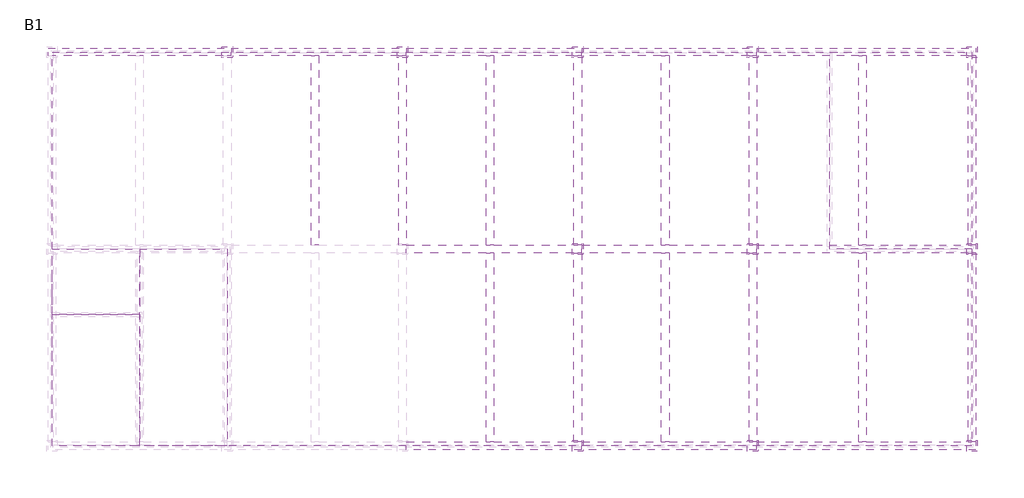
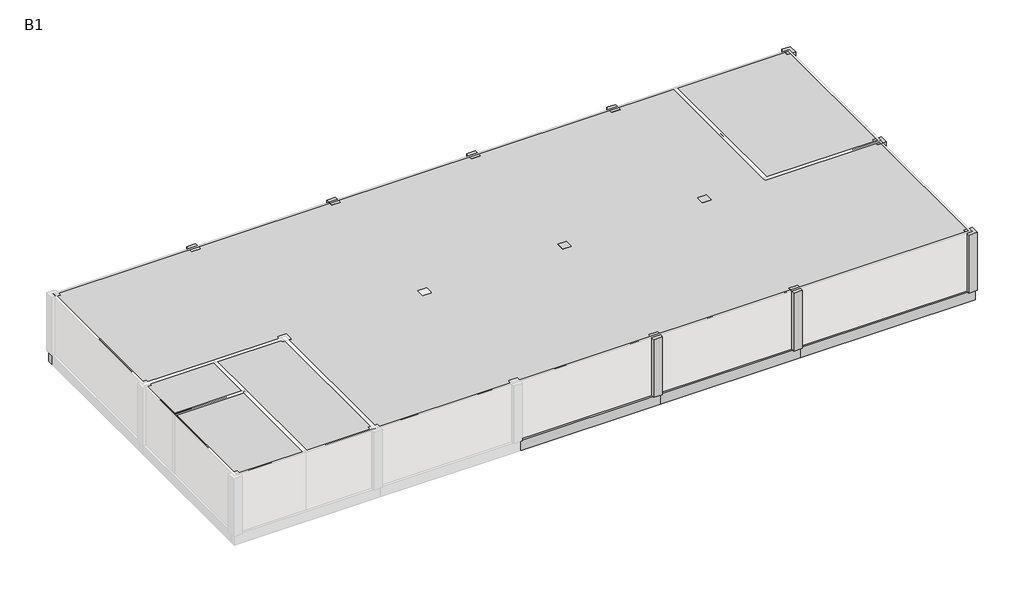
# One storey, part 2 of 2: 25 beams, 11 columns, 5 proxies.
"""IFC4 building model written with IfcOpenShell, lengths in millimetres."""

import ifcopenshell
import ifcopenshell.guid

model = None  # the IFC model being written
_history = None  # IfcOwnerHistory: only IFC2X3 demands one
_inside = {}  # id of a spatial element -> (the spatial element, [elements in it])
_under = {}  # id of a project, library or spatial element -> (it, [spatial elements below it])
_declared = {}  # id of a project -> (the project, [libraries it declares])
_typed = {}  # id of a type object -> (the type object, [elements of that type])
_made_of = {}  # id of a material, layer set ... -> (it, [elements and type objects made of it])


def new_model(schema):
    """Start an empty IFC model of exactly this schema.

    Asked for "IFC4X3", IfcOpenShell would pick the latest addendum, in which some entities
    have other attributes; the version numbers below select the first issue.
    IFC2X3 requires an IfcOwnerHistory on every rooted entity: one is made here for all.
    """
    global model, _history
    if schema == "IFC4X3":
        model = ifcopenshell.file(schema_version=(4, 3, 0, 0))
    else:
        model = ifcopenshell.file(schema=schema)
    _inside.clear()
    _under.clear()
    _declared.clear()
    _typed.clear()
    _made_of.clear()
    _history = None
    if model.schema == "IFC2X3":
        org = make("IfcOrganization", Name="unknown")
        user = make(
            "IfcPersonAndOrganization",
            ThePerson=make("IfcPerson", FamilyName="unknown"),
            TheOrganization=org,
        )
        app = make(
            "IfcApplication",
            ApplicationDeveloper=org,
            Version="unknown",
            ApplicationFullName="unknown",
            ApplicationIdentifier="unknown",
        )
        _history = make(
            "IfcOwnerHistory",
            OwningUser=user,
            OwningApplication=app,
            ChangeAction="ADDED",
            CreationDate=0,
        )
    return model


def make(cls, **values):
    """One entity of the class cls with the attributes given. An attribute that is None is left unset."""
    return model.create_entity(
        cls, **{name: value for name, value in values.items() if value is not None}
    )


def rooted(cls, **values):
    """An entity with a GlobalId (a new one), such as an element, a storey or a relation."""
    return make(cls, GlobalId=ifcopenshell.guid.new(), OwnerHistory=_history, **values)


def si_unit(unit_type, name, prefix=None):
    """IfcSIUnit, for example si_unit("LENGTHUNIT", "METRE", prefix="MILLI")."""
    return make("IfcSIUnit", UnitType=unit_type, Prefix=prefix, Name=name)


def assignment(units):
    """IfcUnitAssignment: the units of a project."""
    return None if units is None else make("IfcUnitAssignment", Units=units)


def point(xyz):
    """IfcCartesianPoint."""
    return None if xyz is None else make("IfcCartesianPoint", Coordinates=xyz)


def direction(xyz):
    """IfcDirection."""
    return None if xyz is None else make("IfcDirection", DirectionRatios=xyz)


def frame(location, z_axis=None, x_axis=None):
    """IfcAxis2Placement3D, a coordinate frame: its origin and axes. An axis left out is left unset."""
    return make(
        "IfcAxis2Placement3D",
        Location=point(location),
        Axis=direction(z_axis),
        RefDirection=direction(x_axis),
    )


def origin():
    """The frame at (0, 0, 0) with its axes left unset."""
    return frame((0.0, 0.0, 0.0))


def origin_with_axes():
    """The frame at (0, 0, 0) with the z axis (0, 0, 1) and the x axis (1, 0, 0) written out."""
    return frame((0.0, 0.0, 0.0), z_axis=(0.0, 0.0, 1.0), x_axis=(1.0, 0.0, 0.0))


def place(relative_to, where):
    """IfcLocalPlacement: puts the frame where relative to a parent placement (None: the world)."""
    return make(
        "IfcLocalPlacement", PlacementRelTo=relative_to, RelativePlacement=where
    )


def context(
    kind, dimensions, precision=None, world=None, true_north=None, identifier=None
):
    """IfcGeometricRepresentationContext, for example the 3D "Model" context."""
    return make(
        "IfcGeometricRepresentationContext",
        ContextIdentifier=identifier,
        ContextType=kind,
        CoordinateSpaceDimension=dimensions,
        Precision=precision,
        WorldCoordinateSystem=world,
        TrueNorth=true_north,
    )


def project(units=None, contexts=None):
    """IfcProject with its units and contexts."""
    return rooted(
        "IfcProject",
        Name="project",
        RepresentationContexts=contexts,
        UnitsInContext=assignment(units),
    )


def spatial(cls, under=None, at=None, **own):
    """A site, building, storey or space (cls), placed at a placement, below another one or the project."""
    s = rooted(cls, ObjectPlacement=at, **own)
    if under is not None:
        _under.setdefault(under.id(), (under, []))[1].append(s)
    return s


def polyline(points):
    """IfcPolyline through the points."""
    return make("IfcPolyline", Points=[point(p) for p in points])


def outline(outer, holes=None, kind="AREA"):
    """IfcArbitraryClosedProfileDef: a profile drawn as a closed curve; with holes, ...WithVoids."""
    if holes is None:
        return make("IfcArbitraryClosedProfileDef", ProfileType=kind, OuterCurve=outer)
    return make(
        "IfcArbitraryProfileDefWithVoids",
        ProfileType=kind,
        OuterCurve=outer,
        InnerCurves=holes,
    )


def extrude(swept, where, along, depth):
    """IfcExtrudedAreaSolid: the profile swept, set in the frame where, extruded along a direction by depth."""
    return make(
        "IfcExtrudedAreaSolid",
        SweptArea=swept,
        Position=where,
        ExtrudedDirection=direction(along),
        Depth=depth,
    )


def faces_of(points, faces, orient=None, outer=None):
    """IfcFace entities. A face is a list of loops; a loop is a list of indices into points, from 0.

    orient and outer hold one flag for each loop. By default every Orientation is true, the
    first loop of a face is its IfcFaceOuterBound and the others are IfcFaceBound.
    """
    made = []
    for i, loops in enumerate(faces):
        bounds = []
        for j, loop in enumerate(loops):
            is_outer = j == 0 if outer is None else outer[i][j]
            bounds.append(
                make(
                    "IfcFaceOuterBound" if is_outer else "IfcFaceBound",
                    Bound=make("IfcPolyLoop", Polygon=[points[k] for k in loop]),
                    Orientation=True if orient is None else orient[i][j],
                )
            )
        made.append(make("IfcFace", Bounds=bounds))
    return made


def faceted_brep(points, faces, orient=None, outer=None, voids=None):
    """IfcFacetedBrep: a solid bounded by flat faces; with voids (closed shells), ...WithVoids."""
    shared = [point(p) for p in points]
    hull = make("IfcClosedShell", CfsFaces=faces_of(shared, faces, orient, outer))
    if voids is None:
        return make("IfcFacetedBrep", Outer=hull)
    return make(
        "IfcFacetedBrepWithVoids",
        Outer=hull,
        Voids=[
            make(cls, CfsFaces=faces_of(shared, fs, o, b)) for cls, fs, o, b in voids
        ],
    )


def shape(context_of_items, identifier, shape_type, items):
    """IfcShapeRepresentation: the items that make up one representation, for example the "Body"."""
    return make(
        "IfcShapeRepresentation",
        ContextOfItems=context_of_items,
        RepresentationIdentifier=identifier,
        RepresentationType=shape_type,
        Items=items,
    )


def source(mapping_origin, context_of_items, identifier, shape_type, items):
    """IfcRepresentationMap: a shape defined once, which mapped items show again and again."""
    return make(
        "IfcRepresentationMap",
        MappingOrigin=mapping_origin,
        MappedRepresentation=shape(context_of_items, identifier, shape_type, items),
    )


def transform(
    local_origin,
    x_axis=None,
    y_axis=None,
    z_axis=None,
    scale=None,
    scale2=None,
    scale3=None,
    uniform=True,
):
    """IfcCartesianTransformationOperator3D, or its non-uniform kind. x_axis, y_axis, z_axis: its Axis1, 2, 3."""
    if uniform:
        return make(
            "IfcCartesianTransformationOperator3D",
            Axis1=direction(x_axis),
            Axis2=direction(y_axis),
            LocalOrigin=point(local_origin),
            Scale=scale,
            Axis3=direction(z_axis),
        )
    return make(
        "IfcCartesianTransformationOperator3DnonUniform",
        Axis1=direction(x_axis),
        Axis2=direction(y_axis),
        LocalOrigin=point(local_origin),
        Scale=scale,
        Axis3=direction(z_axis),
        Scale2=scale2,
        Scale3=scale3,
    )


def mapped(mapping_source, mapping_target):
    """IfcMappedItem: shows the shape of a source again, moved by a transform."""
    return make(
        "IfcMappedItem", MappingSource=mapping_source, MappingTarget=mapping_target
    )


def made_of(thing, what):
    """Note that an element or type object is made of a material, layer set ...; save() writes the relation."""
    if what is not None:
        _made_of.setdefault(what.id(), (what, []))[1].append(thing)
    return thing


def element(
    cls,
    number,
    at=None,
    inside=None,
    cuts=None,
    type_object=None,
    material=None,
    context=None,
    identifier="Body",
    shape_type=None,
    held_by="IfcProductDefinitionShape",
    body=None,
    shapes=None,
    **own,
):
    """One element of the class cls, such as IfcWall. Its Tag is "e" and its number.

    at: its placement. inside: the storey or other place that contains it. cuts: it is an
    opening in that element (IfcRelVoidsElement). A single representation is given by context,
    identifier, shape_type and body (its items); several are given by shapes. held_by: the class
    of the entity that holds the representations. save() writes the other relations.
    """
    e = rooted(cls, Tag="e%d" % number, ObjectPlacement=at, **own)
    if body is not None:
        shapes = [shape(context, identifier, shape_type, body)]
    if shapes is not None:
        e.Representation = make(held_by, Representations=shapes)
    if inside is not None:
        _inside.setdefault(inside.id(), (inside, []))[1].append(e)
    if cuts is not None:
        rooted(
            "IfcRelVoidsElement", RelatingBuildingElement=cuts, RelatedOpeningElement=e
        )
    if type_object is not None:
        _typed.setdefault(type_object.id(), (type_object, []))[1].append(e)
    return made_of(e, material)


def aggregate(whole, parts):
    """IfcRelAggregates: a whole, such as a stair, and the parts it consists of."""
    return rooted("IfcRelAggregates", RelatingObject=whole, RelatedObjects=parts)


def save(model, path):
    """Write the relations noted so far, then the file.

    IfcRelAggregates (storeys below a building ...), IfcRelContainedInSpatialStructure (elements
    in a storey), IfcRelDefinesByType, IfcRelAssociatesMaterial and IfcRelDeclares: one each for
    every whole, place, type object, material and project.
    """
    for whole, parts in _under.values():
        aggregate(whole, parts)
    for where, things in _inside.values():
        rooted(
            "IfcRelContainedInSpatialStructure",
            RelatedElements=things,
            RelatingStructure=where,
        )
    for kind, things in _typed.values():
        rooted("IfcRelDefinesByType", RelatedObjects=things, RelatingType=kind)
    for what, things in _made_of.values():
        rooted("IfcRelAssociatesMaterial", RelatedObjects=things, RelatingMaterial=what)
    for by, libraries in _declared.values():
        rooted("IfcRelDeclares", RelatingContext=by, RelatedDefinitions=libraries)
    model.write(path)


def generic_models_bb515c93(model_context):
    return source(origin(), model_context, "Body", "SweptSolid", [
        extrude(outline(polyline([(9000.0, 21000.0), (9000.0, -21000.0), (-9000.0, -21000.0), (-9000.0, 21000.0), (9000.0, 21000.0)])), origin_with_axes(), (0.0, 0.0, 1.0), 3500.0),
    ])


def generic_models_5926095e(model_context):
    return source(origin(), model_context, "Body", "SweptSolid", [
        extrude(outline(polyline([(3250.0, 4500.0), (3250.0, -4500.0), (-3250.0, -4500.0), (-3250.0, 4500.0), (3250.0, 4500.0)])), origin_with_axes(), (0.0, 0.0, 1.0), 3500.0),
    ])


def generic_models_0b067365(model_context):
    return source(origin(), model_context, "Body", "SweptSolid", [
        extrude(outline(polyline([(2000.0, 4500.0), (2000.0, -4500.0), (-2000.0, -4500.0), (-2000.0, 4500.0), (2000.0, 4500.0)])), origin_with_axes(), (0.0, 0.0, 1.0), 3500.0),
    ])


def generic_models_4c644d41(model_context):
    return source(origin(), model_context, "Body", "SweptSolid", [
        extrude(outline(polyline([(2000.0, 1500.0), (2000.0, -1500.0), (-2000.0, -1500.0), (-2000.0, 1500.0), (2000.0, 1500.0)])), origin_with_axes(), (0.0, 0.0, 1.0), 3500.0),
    ])


def generic_models_c89eb543(model_context):
    return source(origin(), model_context, "Body", "SweptSolid", [
        extrude(outline(polyline([(2000.0, 3000.0), (2000.0, -3000.0), (-2000.0, -3000.0), (-2000.0, 3000.0), (2000.0, 3000.0)])), origin_with_axes(), (0.0, 0.0, 1.0), 3500.0),
    ])


model = new_model("IFC4")

# Units and contexts
model_context = context("Model", 3, world=origin())
ifc_project = project(units=[si_unit("LENGTHUNIT", "METRE", prefix="MILLI")], contexts=[model_context])

# Site, building, storey
site = spatial("IfcSite", under=ifc_project)
building = spatial("IfcBuilding", under=site)
storey = spatial("IfcBuildingStorey", under=building, Name="B1", Elevation=-4000.0)

# Beams
placement = place(None, origin())
element("IfcBeam", 1, ObjectType="Concrete-Rectangular-Beam : BM111_400x500_RG1", at=placement, inside=storey, context=model_context, shape_type="SweptSolid", body=[
    extrude(outline(polyline([(57634.6521483, 173098.8614395), (57284.6521483, 173098.8614395), (57284.6521483, 181748.8614395), (57634.6521483, 181748.8614395), (57634.6521483, 173098.8614395)])), frame((0.0, 0.0, -600.0), z_axis=(0.0, 0.0, 1.0), x_axis=(1.0, 0.0, 0.0)), (0.0, 0.0, 1.0), 600.0),
])
element("IfcBeam", 2, ObjectType="Concrete-Rectangular-Beam : BM111_400x500_RG1", at=placement, inside=storey, context=model_context, shape_type="SweptSolid", body=[
    extrude(outline(polyline([(65634.6521483, 173098.8614395), (65284.6521483, 173098.8614395), (65284.6521483, 181748.8614395), (65634.6521483, 181748.8614395), (65634.6521483, 173098.8614395)])), frame((0.0, 0.0, -600.0), z_axis=(0.0, 0.0, 1.0), x_axis=(1.0, 0.0, 0.0)), (0.0, 0.0, 1.0), 600.0),
])
element("IfcBeam", 3, ObjectType="Concrete-Rectangular-Beam : BM111_400x500_RG1", at=placement, inside=storey, context=model_context, shape_type="SweptSolid", body=[
    extrude(outline(polyline([(65284.6521483, 172748.8614395), (65634.6521483, 172748.8614395), (65634.6521483, 164098.8614395), (65284.6521483, 164098.8614395), (65284.6521483, 172748.8614395)])), frame((0.0, 0.0, -600.0), z_axis=(0.0, 0.0, 1.0), x_axis=(1.0, 0.0, 0.0)), (0.0, 0.0, 1.0), 600.0),
])
element("IfcBeam", 4, ObjectType="Concrete-Rectangular-Beam : BM111_400x500_RG1", at=placement, inside=storey, context=model_context, shape_type="SweptSolid", body=[
    extrude(outline(polyline([(73634.6521483, 173098.8614395), (73284.6521483, 173098.8614395), (73284.6521483, 181748.8614395), (73634.6521483, 181748.8614395), (73634.6521483, 173098.8614395)])), frame((0.0, 0.0, -600.0), z_axis=(0.0, 0.0, 1.0), x_axis=(1.0, 0.0, 0.0)), (0.0, 0.0, 1.0), 600.0),
])
element("IfcBeam", 5, ObjectType="Concrete-Rectangular-Beam : BM111_400x500_RG1", at=placement, inside=storey, context=model_context, shape_type="SweptSolid", body=[
    extrude(outline(polyline([(73284.6521483, 172748.8614395), (73634.6521483, 172748.8614395), (73634.6521483, 164098.8614395), (73284.6521483, 164098.8614395), (73284.6521483, 172748.8614395)])), frame((0.0, 0.0, -600.0), z_axis=(0.0, 0.0, 1.0), x_axis=(1.0, 0.0, 0.0)), (0.0, 0.0, 1.0), 600.0),
])
element("IfcBeam", 6, ObjectType="Concrete-Rectangular-Beam : BM111_400x500_RG1", at=placement, inside=storey, context=model_context, shape_type="SweptSolid", body=[
    extrude(outline(polyline([(82634.6521483, 173098.8614395), (82284.6521483, 173098.8614395), (82284.6521483, 181748.8614395), (82634.6521483, 181748.8614395), (82634.6521483, 173098.8614395)])), frame((0.0, 0.0, -600.0), z_axis=(0.0, 0.0, 1.0), x_axis=(1.0, 0.0, 0.0)), (0.0, 0.0, 1.0), 600.0),
])
element("IfcBeam", 7, ObjectType="Concrete-Rectangular-Beam : BM111_400x500_RG1", at=placement, inside=storey, context=model_context, shape_type="SweptSolid", body=[
    extrude(outline(polyline([(82284.6521483, 172748.8614395), (82634.6521483, 172748.8614395), (82634.6521483, 164098.8614395), (82284.6521483, 164098.8614395), (82284.6521483, 172748.8614395)])), frame((0.0, 0.0, -600.0), z_axis=(0.0, 0.0, 1.0), x_axis=(1.0, 0.0, 0.0)), (0.0, 0.0, 1.0), 600.0),
])
element("IfcBeam", 8, ObjectType="Concrete-Rectangular-Beam : BM111_400x500_RG1", at=placement, inside=storey, context=model_context, shape_type="Brep", body=[
    faceted_brep([(53634.6521483, 181748.8614395, 0.0), (53634.6521483, 182098.8614395, 0.0), (45284.6521483, 182098.8614395, 0.0), (45284.6521483, 181748.8614395, 0.0), (45634.6521483, 181748.8614395, 0.0), (49284.6521483, 181748.8614395, 0.0), (49634.6521483, 181748.8614395, 0.0), (53284.6521483, 181748.8614395, 0.0), (53634.6521483, 181748.8614395, -600.0), (45284.6521483, 181748.8614395, -600.0), (45634.6521483, 181748.8614395, -600.0), (49284.6521483, 181748.8614395, -600.0), (49634.6521483, 181748.8614395, -600.0), (53284.6521483, 181748.8614395, -600.0), (53634.6521483, 182098.8614395, -600.0), (45284.6521483, 182098.8614395, -600.0)], [[[0, 1, 2, 3, 4, 5, 6, 7]], [[8, 0, 7, 6, 5, 4, 3, 9, 10, 11, 12, 13]], [[14, 8, 13, 12, 11, 10, 9, 15]], [[1, 14, 15, 2]], [[1, 0, 8, 14]], [[3, 2, 15, 9]]]),
])
element("IfcBeam", 9, ObjectType="Concrete-Rectangular-Beam : BM111_400x500_RG1", at=placement, inside=storey, context=model_context, shape_type="Brep", body=[
    faceted_brep([(61634.6521483, 181748.8614395, 0.0), (61634.6521483, 182098.8614395, 0.0), (53634.6521483, 182098.8614395, 0.0), (53634.6521483, 181748.8614395, 0.0), (57284.6521483, 181748.8614395, 0.0), (57634.6521483, 181748.8614395, 0.0), (61284.6521483, 181748.8614395, 0.0), (61634.6521483, 181748.8614395, -600.0), (53634.6521483, 181748.8614395, -600.0), (57284.6521483, 181748.8614395, -600.0), (57634.6521483, 181748.8614395, -600.0), (61284.6521483, 181748.8614395, -600.0), (61634.6521483, 182098.8614395, -600.0), (53634.6521483, 182098.8614395, -600.0)], [[[0, 1, 2, 3, 4, 5, 6]], [[7, 0, 6, 5, 4, 3, 8, 9, 10, 11]], [[12, 7, 11, 10, 9, 8, 13]], [[1, 12, 13, 2]], [[1, 0, 7, 12]], [[3, 2, 13, 8]]]),
])
element("IfcBeam", 10, ObjectType="Concrete-Rectangular-Beam : BM111_400x500_RG1", at=placement, inside=storey, context=model_context, shape_type="Brep", body=[
    faceted_brep([(69634.6521483, 181748.8614395, 0.0), (69634.6521483, 182098.8614395, 0.0), (61634.6521483, 182098.8614395, 0.0), (61634.6521483, 181748.8614395, 0.0), (65284.6521483, 181748.8614395, 0.0), (65634.6521483, 181748.8614395, 0.0), (69284.6521483, 181748.8614395, 0.0), (69634.6521483, 181748.8614395, -600.0), (61634.6521483, 181748.8614395, -600.0), (65284.6521483, 181748.8614395, -600.0), (65634.6521483, 181748.8614395, -600.0), (69284.6521483, 181748.8614395, -600.0), (69634.6521483, 182098.8614395, -600.0), (61634.6521483, 182098.8614395, -600.0)], [[[0, 1, 2, 3, 4, 5, 6]], [[7, 0, 6, 5, 4, 3, 8, 9, 10, 11]], [[12, 7, 11, 10, 9, 8, 13]], [[1, 12, 13, 2]], [[1, 0, 7, 12]], [[3, 2, 13, 8]]]),
])
element("IfcBeam", 11, ObjectType="Concrete-Rectangular-Beam : BM111_400x500_RG1", at=placement, inside=storey, context=model_context, shape_type="Brep", body=[
    faceted_brep([(77634.6521483, 181748.8614395, 0.0), (77634.6521483, 182098.8614395, 0.0), (69634.6521483, 182098.8614395, 0.0), (69634.6521483, 181748.8614395, 0.0), (73284.6521483, 181748.8614395, 0.0), (73634.6521483, 181748.8614395, 0.0), (77284.6521483, 181748.8614395, 0.0), (77634.6521483, 181748.8614395, -600.0), (69634.6521483, 181748.8614395, -600.0), (73284.6521483, 181748.8614395, -600.0), (73634.6521483, 181748.8614395, -600.0), (77284.6521483, 181748.8614395, -600.0), (77634.6521483, 182098.8614395, -600.0), (69634.6521483, 182098.8614395, -600.0)], [[[0, 1, 2, 3, 4, 5, 6]], [[7, 0, 6, 5, 4, 3, 8, 9, 10, 11]], [[12, 7, 11, 10, 9, 8, 13]], [[1, 12, 13, 2]], [[1, 0, 7, 12]], [[3, 2, 13, 8]]]),
])
element("IfcBeam", 12, ObjectType="Concrete-Rectangular-Beam : BM111_400x500_RG1", at=placement, inside=storey, context=model_context, shape_type="Brep", body=[
    faceted_brep([(87634.6521483, 181748.8614395, 0.0), (87634.6521483, 182098.8614395, 0.0), (77634.6521483, 182098.8614395, 0.0), (77634.6521483, 181748.8614395, 0.0), (82284.6521483, 181748.8614395, 0.0), (82634.6521483, 181748.8614395, 0.0), (87284.6521483, 181748.8614395, 0.0), (87634.6521483, 181748.8614395, -600.0), (77634.6521483, 181748.8614395, -600.0), (82284.6521483, 181748.8614395, -600.0), (82634.6521483, 181748.8614395, -600.0), (87284.6521483, 181748.8614395, -600.0), (87634.6521483, 182098.8614395, -600.0), (77634.6521483, 182098.8614395, -600.0)], [[[0, 1, 2, 3, 4, 5, 6]], [[7, 0, 6, 5, 4, 3, 8, 9, 10, 11]], [[12, 7, 11, 10, 9, 8, 13]], [[1, 12, 13, 2]], [[1, 0, 7, 12]], [[3, 2, 13, 8]]]),
])
element("IfcBeam", 13, ObjectType="Concrete-Rectangular-Beam : BM111_400x500_RG1", at=placement, inside=storey, context=model_context, shape_type="Brep", body=[
    faceted_brep([(69634.6521483, 172748.8614395, 0.0), (69634.6521483, 173098.8614395, 0.0), (69284.6521483, 173098.8614395, 0.0), (65634.6521483, 173098.8614395, 0.0), (65284.6521483, 173098.8614395, 0.0), (61634.6521483, 173098.8614395, 0.0), (61634.6521483, 172748.8614395, 0.0), (65284.6521483, 172748.8614395, 0.0), (65634.6521483, 172748.8614395, 0.0), (69284.6521483, 172748.8614395, 0.0), (69634.6521483, 172748.8614395, -600.0), (61634.6521483, 172748.8614395, -600.0), (65284.6521483, 172748.8614395, -600.0), (65634.6521483, 172748.8614395, -600.0), (69284.6521483, 172748.8614395, -600.0), (69634.6521483, 173098.8614395, -600.0), (61634.6521483, 173098.8614395, -600.0), (65284.6521483, 173098.8614395, -600.0), (65634.6521483, 173098.8614395, -600.0), (69284.6521483, 173098.8614395, -600.0)], [[[0, 1, 2, 3, 4, 5, 6, 7, 8, 9]], [[10, 0, 9, 8, 7, 6, 11, 12, 13, 14]], [[15, 10, 14, 13, 12, 11, 16, 17, 18, 19]], [[1, 15, 19, 18, 17, 16, 5, 4, 3, 2]], [[1, 0, 10, 15]], [[6, 5, 16, 11]]]),
])
element("IfcBeam", 14, ObjectType="Concrete-Rectangular-Beam : BM111_400x500_RG1", at=placement, inside=storey, context=model_context, shape_type="Brep", body=[
    faceted_brep([(77634.6521483, 172748.8614395, 0.0), (77634.6521483, 173098.8614395, 0.0), (77284.6521483, 173098.8614395, 0.0), (73634.6521483, 173098.8614395, 0.0), (73284.6521483, 173098.8614395, 0.0), (69634.6521483, 173098.8614395, 0.0), (69634.6521483, 172748.8614395, 0.0), (73284.6521483, 172748.8614395, 0.0), (73634.6521483, 172748.8614395, 0.0), (77284.6521483, 172748.8614395, 0.0), (77634.6521483, 172748.8614395, -600.0), (69634.6521483, 172748.8614395, -600.0), (73284.6521483, 172748.8614395, -600.0), (73634.6521483, 172748.8614395, -600.0), (77284.6521483, 172748.8614395, -600.0), (77634.6521483, 173098.8614395, -600.0), (69634.6521483, 173098.8614395, -600.0), (73284.6521483, 173098.8614395, -600.0), (73634.6521483, 173098.8614395, -600.0), (77284.6521483, 173098.8614395, -600.0)], [[[0, 1, 2, 3, 4, 5, 6, 7, 8, 9]], [[10, 0, 9, 8, 7, 6, 11, 12, 13, 14]], [[15, 10, 14, 13, 12, 11, 16, 17, 18, 19]], [[1, 15, 19, 18, 17, 16, 5, 4, 3, 2]], [[1, 0, 10, 15]], [[6, 5, 16, 11]]]),
])
element("IfcBeam", 15, ObjectType="Concrete-Rectangular-Beam : BM111_400x500_RG1", at=placement, inside=storey, context=model_context, shape_type="Brep", body=[
    faceted_brep([(87634.6521483, 172748.8614395, 0.0), (87634.6521483, 173098.8614395, 0.0), (87284.6521483, 173098.8614395, 0.0), (82634.6521483, 173098.8614395, 0.0), (82284.6521483, 173098.8614395, 0.0), (77634.6521483, 173098.8614395, 0.0), (77634.6521483, 172748.8614395, 0.0), (82284.6521483, 172748.8614395, 0.0), (82634.6521483, 172748.8614395, 0.0), (87284.6521483, 172748.8614395, 0.0), (87634.6521483, 172748.8614395, -600.0), (77634.6521483, 172748.8614395, -600.0), (82284.6521483, 172748.8614395, -600.0), (82634.6521483, 172748.8614395, -600.0), (87284.6521483, 172748.8614395, -600.0), (87634.6521483, 173098.8614395, -600.0), (77634.6521483, 173098.8614395, -600.0), (82284.6521483, 173098.8614395, -600.0), (82634.6521483, 173098.8614395, -600.0), (87284.6521483, 173098.8614395, -600.0)], [[[0, 1, 2, 3, 4, 5, 6, 7, 8, 9]], [[10, 0, 9, 8, 7, 6, 11, 12, 13, 14]], [[15, 10, 14, 13, 12, 11, 16, 17, 18, 19]], [[1, 15, 19, 18, 17, 16, 5, 4, 3, 2]], [[1, 0, 10, 15]], [[6, 5, 16, 11]]]),
])
element("IfcBeam", 16, ObjectType="Concrete-Rectangular-Beam : BM111_400x500_RG1", at=placement, inside=storey, context=model_context, shape_type="Brep", body=[
    faceted_brep([(69634.6521483, 163748.8614395, 0.0), (69634.6521483, 164098.8614395, 0.0), (69284.6521483, 164098.8614395, 0.0), (65634.6521483, 164098.8614395, 0.0), (65284.6521483, 164098.8614395, 0.0), (61634.6521483, 164098.8614395, 0.0), (61634.6521483, 163748.8614395, 0.0), (69634.6521483, 163748.8614395, -600.0), (61634.6521483, 163748.8614395, -600.0), (69634.6521483, 164098.8614395, -600.0), (61634.6521483, 164098.8614395, -600.0), (65284.6521483, 164098.8614395, -600.0), (65634.6521483, 164098.8614395, -600.0), (69284.6521483, 164098.8614395, -600.0)], [[[0, 1, 2, 3, 4, 5, 6]], [[7, 0, 6, 8]], [[9, 7, 8, 10, 11, 12, 13]], [[1, 9, 13, 12, 11, 10, 5, 4, 3, 2]], [[1, 0, 7, 9]], [[6, 5, 10, 8]]]),
])
element("IfcBeam", 17, ObjectType="Concrete-Rectangular-Beam : BM111_400x500_RG1", at=placement, inside=storey, context=model_context, shape_type="Brep", body=[
    faceted_brep([(77634.6521483, 163748.8614395, 0.0), (77634.6521483, 164098.8614395, 0.0), (77284.6521483, 164098.8614395, 0.0), (73634.6521483, 164098.8614395, 0.0), (73284.6521483, 164098.8614395, 0.0), (69634.6521483, 164098.8614395, 0.0), (69634.6521483, 163748.8614395, 0.0), (77634.6521483, 163748.8614395, -600.0), (69634.6521483, 163748.8614395, -600.0), (77634.6521483, 164098.8614395, -600.0), (69634.6521483, 164098.8614395, -600.0), (73284.6521483, 164098.8614395, -600.0), (73634.6521483, 164098.8614395, -600.0), (77284.6521483, 164098.8614395, -600.0)], [[[0, 1, 2, 3, 4, 5, 6]], [[7, 0, 6, 8]], [[9, 7, 8, 10, 11, 12, 13]], [[1, 9, 13, 12, 11, 10, 5, 4, 3, 2]], [[1, 0, 7, 9]], [[6, 5, 10, 8]]]),
])
element("IfcBeam", 18, ObjectType="Concrete-Rectangular-Beam : BM111_400x500_RG1", at=placement, inside=storey, context=model_context, shape_type="Brep", body=[
    faceted_brep([(87634.6521483, 163748.8614395, 0.0), (87634.6521483, 164098.8614395, 0.0), (87284.6521483, 164098.8614395, 0.0), (82634.6521483, 164098.8614395, 0.0), (82284.6521483, 164098.8614395, 0.0), (77634.6521483, 164098.8614395, 0.0), (77634.6521483, 163748.8614395, 0.0), (87634.6521483, 163748.8614395, -600.0), (77634.6521483, 163748.8614395, -600.0), (87634.6521483, 164098.8614395, -600.0), (77634.6521483, 164098.8614395, -600.0), (82284.6521483, 164098.8614395, -600.0), (82634.6521483, 164098.8614395, -600.0), (87284.6521483, 164098.8614395, -600.0)], [[[0, 1, 2, 3, 4, 5, 6]], [[7, 0, 6, 8]], [[9, 7, 8, 10, 11, 12, 13]], [[1, 9, 13, 12, 11, 10, 5, 4, 3, 2]], [[1, 0, 7, 9]], [[6, 5, 10, 8]]]),
])
element("IfcBeam", 19, ObjectType="Concrete-Rectangular-Beam : BM111_400x500_RG1", at=placement, inside=storey, context=model_context, shape_type="SweptSolid", body=[
    extrude(outline(polyline([(61284.6521483, 181748.8614395), (61634.6521483, 181748.8614395), (61634.6521483, 173098.8614395), (61284.6521483, 173098.8614395), (61284.6521483, 181748.8614395)])), frame((0.0, 0.0, -600.0), z_axis=(0.0, 0.0, 1.0), x_axis=(1.0, 0.0, 0.0)), (0.0, 0.0, 1.0), 600.0),
])
element("IfcBeam", 20, ObjectType="Concrete-Rectangular-Beam : BM111_400x500_RG1", at=placement, inside=storey, context=model_context, shape_type="SweptSolid", body=[
    extrude(outline(polyline([(69284.6521483, 181748.8614395), (69634.6521483, 181748.8614395), (69634.6521483, 173098.8614395), (69284.6521483, 173098.8614395), (69284.6521483, 181748.8614395)])), frame((0.0, 0.0, -600.0), z_axis=(0.0, 0.0, 1.0), x_axis=(1.0, 0.0, 0.0)), (0.0, 0.0, 1.0), 600.0),
])
element("IfcBeam", 21, ObjectType="Concrete-Rectangular-Beam : BM111_400x500_RG1", at=placement, inside=storey, context=model_context, shape_type="SweptSolid", body=[
    extrude(outline(polyline([(69284.6521483, 172748.8614395), (69634.6521483, 172748.8614395), (69634.6521483, 164098.8614395), (69284.6521483, 164098.8614395), (69284.6521483, 172748.8614395)])), frame((0.0, 0.0, -600.0), z_axis=(0.0, 0.0, 1.0), x_axis=(1.0, 0.0, 0.0)), (0.0, 0.0, 1.0), 600.0),
])
element("IfcBeam", 22, ObjectType="Concrete-Rectangular-Beam : BM111_400x500_RG1", at=placement, inside=storey, context=model_context, shape_type="SweptSolid", body=[
    extrude(outline(polyline([(77284.6521483, 181748.8614395), (77634.6521483, 181748.8614395), (77634.6521483, 173098.8614395), (77284.6521483, 173098.8614395), (77284.6521483, 181748.8614395)])), frame((0.0, 0.0, -600.0), z_axis=(0.0, 0.0, 1.0), x_axis=(1.0, 0.0, 0.0)), (0.0, 0.0, 1.0), 600.0),
])
element("IfcBeam", 23, ObjectType="Concrete-Rectangular-Beam : BM111_400x500_RG1", at=placement, inside=storey, context=model_context, shape_type="SweptSolid", body=[
    extrude(outline(polyline([(77284.6521483, 172748.8614395), (77634.6521483, 172748.8614395), (77634.6521483, 164098.8614395), (77284.6521483, 164098.8614395), (77284.6521483, 172748.8614395)])), frame((0.0, 0.0, -600.0), z_axis=(0.0, 0.0, 1.0), x_axis=(1.0, 0.0, 0.0)), (0.0, 0.0, 1.0), 600.0),
])
element("IfcBeam", 24, ObjectType="Concrete-Rectangular-Beam : BM111_400x500_RG1", at=placement, inside=storey, context=model_context, shape_type="SweptSolid", body=[
    extrude(outline(polyline([(87284.6521483, 181748.8614395), (87634.6521483, 181748.8614395), (87634.6521483, 173098.8614395), (87284.6521483, 173098.8614395), (87284.6521483, 181748.8614395)])), frame((0.0, 0.0, -600.0), z_axis=(0.0, 0.0, 1.0), x_axis=(1.0, 0.0, 0.0)), (0.0, 0.0, 1.0), 600.0),
])
element("IfcBeam", 25, ObjectType="Concrete-Rectangular-Beam : BM111_400x500_RG1", at=placement, inside=storey, context=model_context, shape_type="SweptSolid", body=[
    extrude(outline(polyline([(87284.6521483, 172748.8614395), (87634.6521483, 172748.8614395), (87634.6521483, 164098.8614395), (87284.6521483, 164098.8614395), (87284.6521483, 172748.8614395)])), frame((0.0, 0.0, -600.0), z_axis=(0.0, 0.0, 1.0), x_axis=(1.0, 0.0, 0.0)), (0.0, 0.0, 1.0), 600.0),
])

# Proxies
generic_models_shape = generic_models_bb515c93(model_context)
element("IfcBuildingElementProxy", 26, Name="Space Planning Box_hec : Space Planning Box_hec", ObjectType="Space Planning Box_hec : Space Planning Box_hec", at=placement, inside=storey, context=model_context, shape_type="MappedRepresentation", body=[
    mapped(generic_models_shape, transform((66459.6521483, 172923.8614395, 0.0), x_axis=(0.0, -1.0, 0.0), y_axis=(1.0, 0.0, 0.0), z_axis=(0.0, 0.0, 1.0))),
])
generic_models_2_shape = generic_models_5926095e(model_context)
element("IfcBuildingElementProxy", 27, Name="Space Planning Box_hec : Space Planning Box_hec", ObjectType="Space Planning Box_hec : Space Planning Box_hec", at=placement, inside=storey, context=model_context, shape_type="MappedRepresentation", body=[
    mapped(generic_models_2_shape, transform((84209.6521483, 177423.8614395, 0.0), x_axis=(1.0, 0.0, 0.0), y_axis=(0.0, 1.0, 0.0), z_axis=(0.0, 0.0, 1.0))),
])
generic_models_3_shape = generic_models_0b067365(model_context)
element("IfcBuildingElementProxy", 28, Name="Space Planning Box_hec : Space Planning Box_hec", ObjectType="Space Planning Box_hec : Space Planning Box_hec", at=placement, inside=storey, context=model_context, shape_type="MappedRepresentation", body=[
    mapped(generic_models_3_shape, transform((51459.6521483, 168423.8614395, 0.0), x_axis=(1.0, 0.0, 0.0), y_axis=(0.0, 1.0, 0.0), z_axis=(0.0, 0.0, 1.0))),
])
generic_models_4_shape = generic_models_4c644d41(model_context)
element("IfcBuildingElementProxy", 29, Name="Space Planning Box_hec : Space Planning Box_hec", ObjectType="Space Planning Box_hec : Space Planning Box_hec", at=placement, inside=storey, context=model_context, shape_type="MappedRepresentation", body=[
    mapped(generic_models_4_shape, transform((47459.6521483, 171423.8614395, 0.0), x_axis=(1.0, 0.0, 0.0), y_axis=(0.0, 1.0, 0.0), z_axis=(0.0, 0.0, 1.0))),
])
generic_models_5_shape = generic_models_c89eb543(model_context)
element("IfcBuildingElementProxy", 30, Name="Space Planning Box_hec : Space Planning Box_hec", ObjectType="Space Planning Box_hec : Space Planning Box_hec", at=placement, inside=storey, context=model_context, shape_type="MappedRepresentation", body=[
    mapped(generic_models_5_shape, transform((47459.6521483, 166923.8614395, 0.0), x_axis=(1.0, 0.0, 0.0), y_axis=(0.0, 1.0, 0.0), z_axis=(0.0, 0.0, 1.0))),
])

# Columns
element("IfcColumn", 31, ObjectType="Concrete-Rectangular-Column : CL111_500x500", at=placement, inside=storey, context=model_context, shape_type="Brep", body=[
    faceted_brep([(53709.6521483, 182173.8614395, 0.0), (53709.6521483, 181673.8614395, 0.0), (53209.6521483, 181673.8614395, 0.0), (53209.6521483, 182173.8614395, 0.0), (53709.6521483, 182173.8614395, 3500.0), (53709.6521483, 182098.8614395, 3500.0), (53709.6521483, 181748.8614395, 3500.0), (53709.6521483, 181673.8614395, 3500.0), (53634.6521483, 181673.8614395, 3500.0), (53284.6521483, 181673.8614395, 3500.0), (53209.6521483, 181673.8614395, 3500.0), (53209.6521483, 181748.8614395, 3500.0), (53209.6521483, 182098.8614395, 3500.0), (53209.6521483, 182173.8614395, 3500.0)], [[[0, 1, 2, 3]], [[4, 5, 6, 7, 1, 0]], [[7, 8, 9, 10, 2, 1]], [[10, 11, 12, 13, 3, 2]], [[13, 4, 0, 3]], [[4, 13, 12, 11, 10, 9, 8, 7, 6, 5]]]),
])
element("IfcColumn", 32, ObjectType="Concrete-Rectangular-Column : CL111_500x500", at=placement, inside=storey, context=model_context, shape_type="Brep", body=[
    faceted_brep([(61709.6521483, 182173.8614395, 0.0), (61709.6521483, 181673.8614395, 0.0), (61209.6521483, 181673.8614395, 0.0), (61209.6521483, 182173.8614395, 0.0), (61709.6521483, 182173.8614395, 3500.0), (61709.6521483, 182098.8614395, 3500.0), (61709.6521483, 181748.8614395, 3500.0), (61709.6521483, 181673.8614395, 3500.0), (61634.6521483, 181673.8614395, 3500.0), (61284.6521483, 181673.8614395, 3500.0), (61209.6521483, 181673.8614395, 3500.0), (61209.6521483, 181748.8614395, 3500.0), (61209.6521483, 182098.8614395, 3500.0), (61209.6521483, 182173.8614395, 3500.0)], [[[0, 1, 2, 3]], [[4, 5, 6, 7, 1, 0]], [[7, 8, 9, 10, 2, 1]], [[10, 11, 12, 13, 3, 2]], [[13, 4, 0, 3]], [[4, 13, 12, 11, 10, 9, 8, 7, 6, 5]]]),
])
element("IfcColumn", 33, ObjectType="Concrete-Rectangular-Column : CL111_500x500", at=placement, inside=storey, context=model_context, shape_type="Brep", body=[
    faceted_brep([(69709.6521483, 182173.8614395, 0.0), (69709.6521483, 181673.8614395, 0.0), (69209.6521483, 181673.8614395, 0.0), (69209.6521483, 182173.8614395, 0.0), (69709.6521483, 182173.8614395, 3500.0), (69709.6521483, 182098.8614395, 3500.0), (69709.6521483, 181748.8614395, 3500.0), (69709.6521483, 181673.8614395, 3500.0), (69634.6521483, 181673.8614395, 3500.0), (69284.6521483, 181673.8614395, 3500.0), (69209.6521483, 181673.8614395, 3500.0), (69209.6521483, 181748.8614395, 3500.0), (69209.6521483, 182098.8614395, 3500.0), (69209.6521483, 182173.8614395, 3500.0)], [[[0, 1, 2, 3]], [[4, 5, 6, 7, 1, 0]], [[7, 8, 9, 10, 2, 1]], [[10, 11, 12, 13, 3, 2]], [[13, 4, 0, 3]], [[4, 13, 12, 11, 10, 9, 8, 7, 6, 5]]]),
])
element("IfcColumn", 34, ObjectType="Concrete-Rectangular-Column : CL111_500x500", at=placement, inside=storey, context=model_context, shape_type="Brep", body=[
    faceted_brep([(77709.6521483, 182173.8614395, 0.0), (77709.6521483, 181673.8614395, 0.0), (77209.6521483, 181673.8614395, 0.0), (77209.6521483, 182173.8614395, 0.0), (77709.6521483, 182173.8614395, 3500.0), (77709.6521483, 182098.8614395, 3500.0), (77709.6521483, 181748.8614395, 3500.0), (77709.6521483, 181673.8614395, 3500.0), (77634.6521483, 181673.8614395, 3500.0), (77284.6521483, 181673.8614395, 3500.0), (77209.6521483, 181673.8614395, 3500.0), (77209.6521483, 181748.8614395, 3500.0), (77209.6521483, 182098.8614395, 3500.0), (77209.6521483, 182173.8614395, 3500.0)], [[[0, 1, 2, 3]], [[4, 5, 6, 7, 1, 0]], [[7, 8, 9, 10, 2, 1]], [[10, 11, 12, 13, 3, 2]], [[13, 4, 0, 3]], [[4, 13, 12, 11, 10, 9, 8, 7, 6, 5]]]),
])
element("IfcColumn", 35, ObjectType="Concrete-Rectangular-Column : CL111_500x500", at=placement, inside=storey, context=model_context, shape_type="Brep", body=[
    faceted_brep([(87709.6521483, 182173.8614395, 0.0), (87709.6521483, 181673.8614395, 0.0), (87209.6521483, 181673.8614395, 0.0), (87209.6521483, 182173.8614395, 0.0), (87709.6521483, 182173.8614395, 3500.0), (87709.6521483, 181673.8614395, 3500.0), (87634.6521483, 181673.8614395, 3500.0), (87284.6521483, 181673.8614395, 3500.0), (87209.6521483, 181673.8614395, 3500.0), (87209.6521483, 181748.8614395, 3500.0), (87209.6521483, 182098.8614395, 3500.0), (87209.6521483, 182173.8614395, 3500.0)], [[[0, 1, 2, 3]], [[4, 5, 1, 0]], [[5, 6, 7, 8, 2, 1]], [[8, 9, 10, 11, 3, 2]], [[11, 4, 0, 3]], [[4, 11, 10, 9, 8, 7, 6, 5]]]),
])
element("IfcColumn", 36, ObjectType="Concrete-Rectangular-Column : CL111_500x500", at=placement, inside=storey, context=model_context, shape_type="Brep", body=[
    faceted_brep([(69709.6521483, 173173.8614395, 0.0), (69709.6521483, 172673.8614395, 0.0), (69209.6521483, 172673.8614395, 0.0), (69209.6521483, 173173.8614395, 0.0), (69709.6521483, 173173.8614395, 3500.0), (69709.6521483, 173098.8614395, 3500.0), (69709.6521483, 172748.8614395, 3500.0), (69709.6521483, 172673.8614395, 3500.0), (69634.6521483, 172673.8614395, 3500.0), (69284.6521483, 172673.8614395, 3500.0), (69209.6521483, 172673.8614395, 3500.0), (69209.6521483, 172748.8614395, 3500.0), (69209.6521483, 173098.8614395, 3500.0), (69209.6521483, 173173.8614395, 3500.0), (69284.6521483, 173173.8614395, 3500.0), (69634.6521483, 173173.8614395, 3500.0)], [[[0, 1, 2, 3]], [[4, 5, 6, 7, 1, 0]], [[7, 8, 9, 10, 2, 1]], [[10, 11, 12, 13, 3, 2]], [[13, 14, 15, 4, 0, 3]], [[4, 15, 14, 13, 12, 11, 10, 9, 8, 7, 6, 5]]]),
])
element("IfcColumn", 37, ObjectType="Concrete-Rectangular-Column : CL111_500x500", at=placement, inside=storey, context=model_context, shape_type="Brep", body=[
    faceted_brep([(77709.6521483, 173173.8614395, 0.0), (77709.6521483, 172673.8614395, 0.0), (77209.6521483, 172673.8614395, 0.0), (77209.6521483, 173173.8614395, 0.0), (77709.6521483, 173173.8614395, 3500.0), (77709.6521483, 173098.8614395, 3500.0), (77709.6521483, 172748.8614395, 3500.0), (77709.6521483, 172673.8614395, 3500.0), (77634.6521483, 172673.8614395, 3500.0), (77284.6521483, 172673.8614395, 3500.0), (77209.6521483, 172673.8614395, 3500.0), (77209.6521483, 172748.8614395, 3500.0), (77209.6521483, 173098.8614395, 3500.0), (77209.6521483, 173173.8614395, 3500.0), (77284.6521483, 173173.8614395, 3500.0), (77634.6521483, 173173.8614395, 3500.0)], [[[0, 1, 2, 3]], [[4, 5, 6, 7, 1, 0]], [[7, 8, 9, 10, 2, 1]], [[10, 11, 12, 13, 3, 2]], [[13, 14, 15, 4, 0, 3]], [[4, 15, 14, 13, 12, 11, 10, 9, 8, 7, 6, 5]]]),
])
element("IfcColumn", 38, ObjectType="Concrete-Rectangular-Column : CL111_500x500", at=placement, inside=storey, context=model_context, shape_type="Brep", body=[
    faceted_brep([(87709.6521483, 173173.8614395, 0.0), (87709.6521483, 172673.8614395, 0.0), (87209.6521483, 172673.8614395, 0.0), (87209.6521483, 173173.8614395, 0.0), (87709.6521483, 173173.8614395, 3500.0), (87709.6521483, 172673.8614395, 3500.0), (87634.6521483, 172673.8614395, 3500.0), (87284.6521483, 172673.8614395, 3500.0), (87209.6521483, 172673.8614395, 3500.0), (87209.6521483, 172748.8614395, 3500.0), (87209.6521483, 173098.8614395, 3500.0), (87209.6521483, 173173.8614395, 3500.0), (87284.6521483, 173173.8614395, 3500.0), (87634.6521483, 173173.8614395, 3500.0)], [[[0, 1, 2, 3]], [[4, 5, 1, 0]], [[5, 6, 7, 8, 2, 1]], [[8, 9, 10, 11, 3, 2]], [[11, 12, 13, 4, 0, 3]], [[4, 13, 12, 11, 10, 9, 8, 7, 6, 5]]]),
])
element("IfcColumn", 39, ObjectType="Concrete-Rectangular-Column : CL111_500x500", at=placement, inside=storey, context=model_context, shape_type="Brep", body=[
    faceted_brep([(69709.6521483, 164173.8614395, 0.0), (69709.6521483, 163673.8614395, 0.0), (69209.6521483, 163673.8614395, 0.0), (69209.6521483, 164173.8614395, 0.0), (69709.6521483, 164173.8614395, 3500.0), (69709.6521483, 164098.8614395, 3500.0), (69709.6521483, 163748.8614395, 3500.0), (69709.6521483, 163673.8614395, 3500.0), (69209.6521483, 163673.8614395, 3500.0), (69209.6521483, 163748.8614395, 3500.0), (69209.6521483, 164098.8614395, 3500.0), (69209.6521483, 164173.8614395, 3500.0), (69284.6521483, 164173.8614395, 3500.0), (69634.6521483, 164173.8614395, 3500.0)], [[[0, 1, 2, 3]], [[4, 5, 6, 7, 1, 0]], [[7, 8, 2, 1]], [[8, 9, 10, 11, 3, 2]], [[11, 12, 13, 4, 0, 3]], [[4, 13, 12, 11, 10, 9, 8, 7, 6, 5]]]),
])
element("IfcColumn", 40, ObjectType="Concrete-Rectangular-Column : CL111_500x500", at=placement, inside=storey, context=model_context, shape_type="Brep", body=[
    faceted_brep([(77709.6521483, 164173.8614395, 0.0), (77709.6521483, 163673.8614395, 0.0), (77209.6521483, 163673.8614395, 0.0), (77209.6521483, 164173.8614395, 0.0), (77709.6521483, 164173.8614395, 3500.0), (77709.6521483, 164098.8614395, 3500.0), (77709.6521483, 163748.8614395, 3500.0), (77709.6521483, 163673.8614395, 3500.0), (77209.6521483, 163673.8614395, 3500.0), (77209.6521483, 163748.8614395, 3500.0), (77209.6521483, 164098.8614395, 3500.0), (77209.6521483, 164173.8614395, 3500.0), (77284.6521483, 164173.8614395, 3500.0), (77634.6521483, 164173.8614395, 3500.0)], [[[0, 1, 2, 3]], [[4, 5, 6, 7, 1, 0]], [[7, 8, 2, 1]], [[8, 9, 10, 11, 3, 2]], [[11, 12, 13, 4, 0, 3]], [[4, 13, 12, 11, 10, 9, 8, 7, 6, 5]]]),
])
element("IfcColumn", 41, ObjectType="Concrete-Rectangular-Column : CL111_500x500", at=placement, inside=storey, context=model_context, shape_type="Brep", body=[
    faceted_brep([(87709.6521483, 164173.8614395, 0.0), (87709.6521483, 163673.8614395, 0.0), (87209.6521483, 163673.8614395, 0.0), (87209.6521483, 164173.8614395, 0.0), (87709.6521483, 164173.8614395, 3500.0), (87709.6521483, 163673.8614395, 3500.0), (87209.6521483, 163673.8614395, 3500.0), (87209.6521483, 163748.8614395, 3500.0), (87209.6521483, 164098.8614395, 3500.0), (87209.6521483, 164173.8614395, 3500.0), (87284.6521483, 164173.8614395, 3500.0), (87634.6521483, 164173.8614395, 3500.0)], [[[0, 1, 2, 3]], [[4, 5, 1, 0]], [[5, 6, 2, 1]], [[6, 7, 8, 9, 3, 2]], [[9, 10, 11, 4, 0, 3]], [[4, 11, 10, 9, 8, 7, 6, 5]]]),
])

save(model, "model.ifc")

# Revit data of these elements
# Type "Concrete-Rectangular-Beam : BM111_400x500_RG1"
#   중앙부 하부근 = "3-D20"
#   중앙부 상부근 = "3-D20"
#   중앙부 보조근 = ""
#   중앙부 늑근 = "2-D10 @200"
#   외단부 하부근 = "3-D20"
#   외단부 상부근 = "3-D20"
#   외단부 보조근 = ""
#   외단부 늑근 = "2-D10 @100"
#   부호 = "RG1"
#   내단부 하부근 = "3-D20"
#   내단부 상부근 = "3-D20"
#   내단부 보조근 = ""
#   내단부 늑근 = "2-D10 @100"
#   ALL 하부근 = ""
#   ALL 상부근 = ""
#   ALL 보조근 = ""
#   ALL 늑근 = ""
#   Width = 400 mm
#   Height = 500 mm
#   Length [instance default] = 1524 mm
#   Structural Material [instance default] = 콘크리트 - 현장타설 콘크리트
#   hec_material3 [instance default] = none
#   hec_material2 [instance default] = none
#   hec_material1 [instance default] = none
#   Assembly Code = ""
# Type "Space Planning Box_hec : Space Planning Box_hec"
#   Type Comments = "..."
#   Room Name [instance default] = "?"
#   Interior Finish [instance default] = ""
#   Exterior Finish [instance default] = ""
#   Department [instance default] = ""
#   Assembly Code = "..."
#   ceiling height [instance default] = 0
#   Width [instance default] = 1524 mm
#   Program Area [instance default] = 0.00 m²
#   Length [instance default] = 1524 mm
#   Height [instance default] = 1524 mm
#   Area [instance default] = 2.32258 m²
#   Fill Color [instance default] = Cyan
#   Default Elevation = 0
# Type "Concrete-Rectangular-Column : CL111_500x500"
#   Description = "UG 철골 기둥용 Pedestal"
#   b = 500 mm
#   h = 500 mm
#   hec_material3 [instance default] = none
#   hec_material2 [instance default] = A03AE056-00001_Bitumen/Bituminous/Asphalt Coating
#   hec_material1 [instance default] = A03AC035-00001_Form Work (3 times in use)_Flat
#   Structural Material [instance default] = A03AC032-00007_Structural Concrete_Type1_25MPa-30Mpa
# Elements 1, 2, 3, 4, 5, 6, 7, 8, 9, 10, 11, 12, 13, 14, 15, 16, 17, 18, 19, 20, 21, 22, 23, 24, 25 (IfcBeam, "Concrete-Rectangular-Beam : BM111_400x500_RG1")
#   Comments = ""
#   hec_material3 = none
#   hec_material2 = none
#   hec_material1 = none
#   Structural Material = 콘크리트 - 현장타설 콘크리트
#   Phase Created = New Construction
#   Materials on its faces: "콘크리트 - 현장타설 콘크리트"
# Element 26 (IfcBuildingElementProxy, "Space Planning Box_hec : Space Planning Box_hec")
#   Room Name = "Cable Room"
#   Interior Finish = "IW5..IW2..N/A,,WK1..N/A,,FL1..N/A,,CL1..N/A"
#   Exterior Finish = "N/A..N/A,,EW1..EW2..N/A"
#   Department = "EL"
#   ceiling height = 0
#   Width = 18000 mm
#   Program Area = 720.00 m²
#   Length = 42000 mm
#   Height = 3500 mm
#   Area = 756.00 m²
#   Fill Color = Orange
#   Phase Created = New Construction
#   Materials on its faces: "Orange"
# Element 27 (IfcBuildingElementProxy, "Space Planning Box_hec : Space Planning Box_hec")
#   Room Name = "Battery Room"
#   Interior Finish = "IW2..N/A..N/A,,N/A..N/A,,FL7..N/A,,CL2..N/A"
#   Exterior Finish = "N/A..N/A,,EW2..N/A..N/A"
#   Department = "EL"
#   ceiling height = 0
#   Width = 6500 mm
#   Program Area = 58.50 m²
#   Length = 9000 mm
#   Height = 3500 mm
#   Area = 58.50 m²
#   Fill Color = Orange
#   Phase Created = New Construction
#   Materials on its faces: "Orange"
# Element 28 (IfcBuildingElementProxy, "Space Planning Box_hec : Space Planning Box_hec")
#   Room Name = "Lobby"
#   Interior Finish = "IW5..N/A..N/A,,WK3..N/A,,FL2..N/A,,N/A..N/A"
#   Exterior Finish = "N/A..N/A,,EW2..N/A..N/A"
#   Department = "AR"
#   ceiling height = 0
#   Width = 4000 mm
#   Program Area = 0.00 m²
#   Length = 9000 mm
#   Height = 3500 mm
#   Area = 36.00 m²
#   Fill Color = Cyan
#   Phase Created = New Construction
#   Materials on its faces: "Cyan"
# Element 29 (IfcBuildingElementProxy, "Space Planning Box_hec : Space Planning Box_hec")
#   Room Name = "Elevator"
#   Interior Finish = "N/A..N/A..N/A,,N/A..N/A,,,,CL3..N/A"
#   Exterior Finish = "N/A..N/A,,EW2..N/A..N/A"
#   Department = "AR"
#   ceiling height = 0
#   Width = 4000 mm
#   Program Area = 0.00 m²
#   Length = 3000 mm
#   Height = 3500 mm
#   Area = 12.00 m²
#   Fill Color = Cyan
#   Phase Created = New Construction
#   Materials on its faces: "Cyan"
# Element 30 (IfcBuildingElementProxy, "Space Planning Box_hec : Space Planning Box_hec")
#   Room Name = "Stairway"
#   Interior Finish = "IW5..N/A..N/A,,WK3..N/A,,FL2..N/A,,CL1..N/A"
#   Exterior Finish = "N/A..N/A,,EW2..N/A..N/A"
#   Department = "PATHV1"
#   ceiling height = 0
#   Width = 4000 mm
#   Program Area = 36.00 m²
#   Length = 6000 mm
#   Height = 3500 mm
#   Area = 24.00 m²
#   Fill Color = Green
#   Phase Created = New Construction
#   Materials on its faces: "Green"
# Elements 31, 32, 33, 34, 35, 36, 37, 38, 39, 40, 41 (IfcColumn, "Concrete-Rectangular-Column : CL111_500x500")
#   Comments = ""
#   hec_material3 = none
#   hec_material2 = none
#   hec_material1 = none
#   Structural Material = 콘크리트 - 현장타설 콘크리트
#   Phase Created = New Construction
#   Materials on its faces: "콘크리트 - 현장타설 콘크리트"
# Materials
#   "콘크리트 - 현장타설 콘크리트": class "콘크리트", colour RGB 192 192 192, transparency 0
#   "Cyan": class "Generic", colour RGB 0 255 255, transparency 0.2, Cost = 0
#   "A03AE056-00001_Bitumen/Bituminous/Asphalt Coating": class "Generic", colour RGB 17 17 17, transparency 0, Description = "Damp-proofing", W00) Work Master Code = "A03AE056-00001", W01) Work Master_Lv1 = "Concrete Work", W02) Work Master_Lv2 = "Concrete Protective Coating (U/G)", W03) Work Master_Spec.1 = "Bitumen/Bituminous/Asphalt Coating", Cost = 0
#   "A03AC035-00001_Form Work (3 times in use)_Flat": class "Wood", colour RGB 149 120 74, transparency 0, Description = "Plywood", W00) Work Master Code = "A03AC035-00001", W01) Work Master_Lv1 = "Concrete Work", W02) Work Master_Lv2 = "Substructure Work", W03) Work Master_Spec.1 = "Form Work (3 times in use)", W04) Work Master_Spec.2 = "Flat Form", W05) Work Master_Spec.3 = "Dressed Lumber, Plywood or Steel Form(Wood Planks are not Allowed) incl. Chamfer", Cost = 0
#   "A03AC032-00007_Structural Concrete_Type1_25MPa-30Mpa": class "Concrete", colour RGB 176 176 176, transparency 0, Keynote = "09910.A1", Description = "Reinf. Conc.", W00) Work Master Code = "A03AC032-00007", W01) Work Master_Lv1 = "Concrete Work", W02) Work Master_Lv2 = "Substructure Work", W03) Work Master_Spec.1 = "Structural Concrete", W04) Work Master_Spec.2 = "Cement Type-1", W05) Work Master_Spec.3 = "25MPa < F'c (Cylinder Strength) ≤ 30MPa", Cost = 0
#   "Orange": class "Generic", colour RGB 255 165 0, transparency 0.2, Cost = 0
#   "Green": class "Generic", colour RGB 0 128 0, transparency 0.2, Cost = 0
